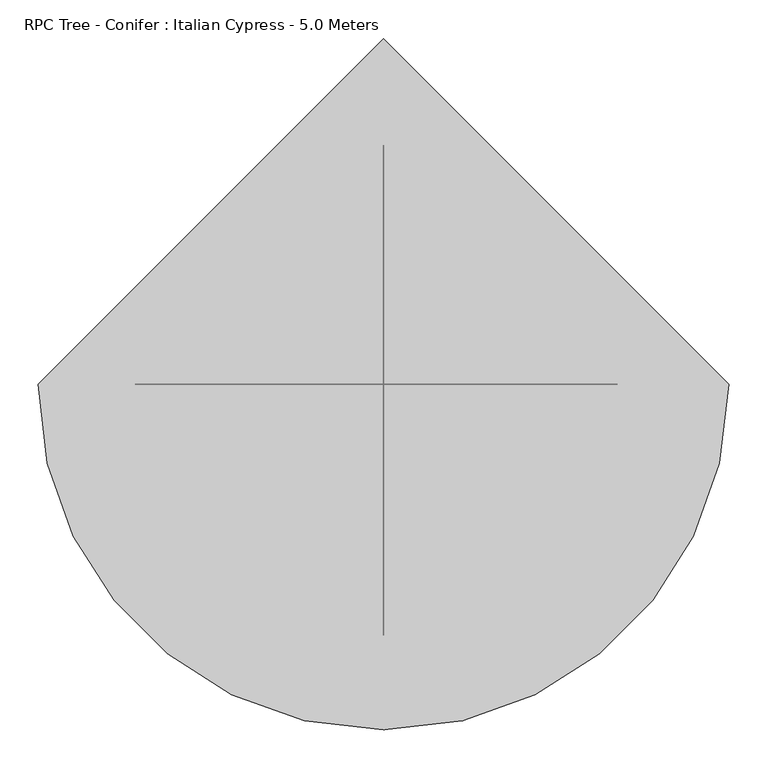
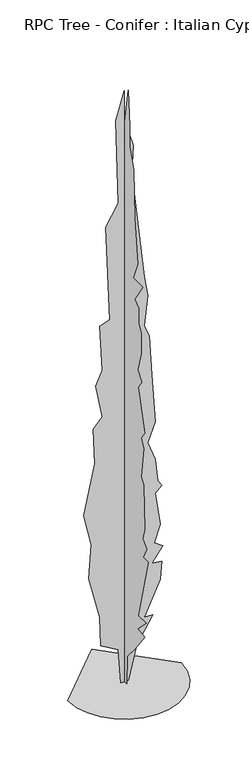
"""IFC4 building model written with IfcOpenShell, lengths in millimetres: geographic element geometry, RPC Tree - Conifer : Italian Cypress - 5.0 Meters."""

from ifc_helpers import new_model, si_unit, origin, place, context, project, spatial, triangles, source, transform, mapped, element, save


def rpc_tree_conifer_italian_cypress_5_0_meters_fed229bb(model_context):
    return source(origin(), model_context, "Body", "Tessellation", [
        triangles([(-28.9243291, 1.3e-06, 0.1175505), (-48.5995771, -1.5e-05, 287.7924989), (-186.3258362, -1.37e-05, 366.4949987), (-196.1633353, -2.79e-05, 612.4350014), (-284.7008453, -4.52e-05, 966.5875122), (-265.0258471, -6.24e-05, 1242.0400303), (-324.0508235, -7.57e-05, 1507.6550674), (-235.513586, -0.0001036, 1910.9949829), (-245.3513394, -0.0001208, 2206.125079), (-176.4880827, -0.0001285, 2284.8250717), (-225.6760869, -0.0001427, 2560.275119), (-176.4880827, -0.0001519, 2678.3248901), (-196.1633353, -0.0001733, 3052.1500374), (-117.4625795, -0.0001785, 3081.6749794), (-146.9753311, -0.0002242, 3868.6749069), (-48.5993273, -0.0002384, 4035.9251633), (-68.2745799, -0.0002792, 4734.3749725), (0.5886036, -0.0002957, 4960.6501144), (0.5885936, -0.0002816, 4724.5499908), (69.4516746, -0.00027, 4478.6001778), (59.614171, -0.0002561, 4252.3500343), (157.9899204, -0.0002064, 3347.2750465), (187.5026721, -0.0001977, 3180.0500793), (157.9899204, -0.0001818, 2934.0999756), (197.3401711, -0.0001776, 2835.7251663), (217.0154237, -0.0001586, 2501.2499428), (246.5281571, -0.0001358, 2097.9100273), (187.5026721, -0.0001239, 1940.5100418), (246.5281571, -0.000117, 1783.1075855), (266.2041727, -0.0001068, 1596.1925411), (295.71667, -0.0001051, 1547.0049911), (246.5281571, -0.0001, 1497.8174412), (285.8791709, -8.53e-05, 1222.3650684), (236.690658, -7.5e-05, 1084.6375013), (305.5541691, -7.51e-05, 1035.450024), (217.0154237, -6.42e-05, 917.4000349), (295.71667, -6.7e-05, 907.5624813), (285.8791709, -5.78e-05, 759.997506), (157.9899204, -3.58e-05, 484.5449879), (226.8529228, -3.88e-05, 484.5449879), (98.9641719, -2.09e-05, 277.9549998), (30.1011696, -1.3e-06, 0.058986), (0.1966738, 26.4907499, 3.55e-05), (0.1966807, 16.6530749, 238.6054939), (0.196685, 95.3537546, 258.2800016), (0.196697, 203.5672438, 494.3825051), (0.1967129, 311.7799882, 819.0225368), (0.1967124, 233.0799954, 887.8875195), (0.1967188, 242.9174945, 1094.4749823), (0.1967282, 272.43001, 1419.1174484), (0.1967333, 262.5925109, 1547.0049911), (0.1967324, 213.4047429, 1645.3799458), (0.1967414, 272.43001, 1861.8075783), (0.1967478, 193.7295085, 2156.9350582), (0.196749, 174.0545104, 2274.9874454), (0.1967577, 223.2422602, 2422.54995), (0.1967593, 164.2167569, 2658.6499283), (0.1967653, 174.054256, 2786.5499702), (0.1967665, 134.7040053, 2924.2749939), (0.1967759, 154.3792578, 3189.875061), (0.1967755, 85.5160011, 3317.775103), (0.1967853, 124.8664971, 3504.675032), (0.19679, 75.678502, 3799.8250397), (0.1967981, 36.3279992, 4094.9500488), (0.1968071, 65.8407486, 4340.8751541), (0.1968079, 26.4905001, 4468.7749054), (0.1968139, -3.0223, 4704.875029), (0.1968216, -52.2102488, 5000.0000381), (0.1968108, -71.8855014, 4704.875029), (0.1968066, -71.8855014, 4537.6250633), (0.1968002, -130.9110046, 4380.2250778), (0.1967852, -140.7485037, 3976.899987), (0.1967737, -180.0987453, 3612.9001122), (0.1967729, -121.0732512, 3465.3251083), (0.1967673, -248.962002, 3465.3251083), (0.1967647, -140.7485037, 3298.1001411), (0.1967635, -199.7739979, 3258.7499268), (0.1967579, -199.7739979, 3130.8498848), (0.1967536, -229.2867495, 3062.0000175), (0.1967493, -229.2867495, 2894.7500519), (0.1967472, -180.0987453, 2727.5250847), (0.1967416, -239.1242486, 2658.6499283), (0.1967438, -189.9364988, 2589.800061), (0.1967284, -278.475008, 2255.3124836), (0.1967275, -229.2867495, 2186.4499718), (0.1967259, -268.6375089, 2117.5849892), (0.1967195, -229.2867495, 1861.8075783), (0.1967156, -268.6375089, 1812.6200283), (0.1967054, -278.475008, 1448.6300365), (0.1967024, -248.9617477, 1350.2524658), (0.1966976, -307.9874871, 1301.0650612), (0.1966986, -258.8000098, 1202.6900339), (0.1966956, -327.6624853, 1202.6900339), (0.1966845, -189.9362444, 671.4600323), (0.1966797, -298.1500062, 671.4600323), (0.1966828, -180.0987453, 553.4074997), (0.1966781, -278.475008, 543.5700188), (0.196679, -150.5860028, 366.4949987), (0.1966781, -42.3724999, 238.6054939), (0.1966712, -32.534751, 3.2e-05), (-450.413314, 0.0, 5.36e-05), (-438.5008143, -103.2502475, 4.7e-05), (-404.5758139, -198.0692509, 3.98e-05), (-351.3483215, -281.7399977, 3.25e-05), (-281.5433345, -351.54751, 2.53e-05), (-197.8723334, -404.7699881, 1.85e-05), (-103.0535753, -438.6974957, 1.23e-05), (0.1966927, -450.6125024, 7.1e-06), (103.4469197, -438.6974957, 3.3e-06), (198.2659141, -404.7724952, 1.1e-06), (281.9366608, -351.5450028, 7e-07), (351.7441913, -281.7399977, 1.8e-06), (404.9666694, -198.0689966, 4.4e-06), (438.894177, -103.2502475, 8.6e-06), (450.8066766, 3.94e-05, 1.42e-05), (0.1966127, 450.6125024, 6.08e-05)], [[17, 18, 19], [39, 40, 41], [16, 17, 19], [16, 19, 20], [16, 20, 21], [16, 21, 22], [15, 16, 22], [14, 15, 22], [14, 22, 23], [14, 23, 24], [34, 35, 36], [36, 37, 38], [42, 1, 2], [41, 42, 2], [39, 41, 2], [30, 31, 32], [39, 2, 3], [39, 3, 4], [38, 39, 4], [36, 38, 4], [36, 4, 5], [34, 36, 5], [34, 5, 6], [33, 34, 6], [32, 33, 6], [32, 6, 7], [32, 7, 8], [30, 32, 8], [29, 30, 8], [28, 29, 8], [28, 8, 9], [27, 28, 9], [27, 9, 10], [26, 27, 10], [26, 10, 11], [26, 11, 12], [25, 26, 12], [25, 12, 13], [24, 25, 13], [14, 24, 13], [67, 68, 69], [94, 95, 96], [74, 75, 76], [96, 97, 98], [92, 93, 94], [100, 43, 44], [99, 100, 44], [67, 69, 70], [66, 67, 70], [66, 70, 71], [65, 66, 71], [65, 71, 72], [64, 65, 72], [63, 64, 72], [63, 72, 73], [62, 63, 73], [62, 73, 74], [61, 62, 74], [61, 74, 76], [90, 91, 92], [81, 82, 83], [46, 47, 48], [60, 61, 76], [59, 60, 76], [59, 76, 77], [59, 77, 78], [59, 78, 79], [59, 79, 80], [59, 80, 81], [58, 59, 81], [57, 58, 81], [57, 81, 83], [56, 57, 83], [56, 83, 84], [55, 56, 84], [55, 84, 85], [54, 55, 85], [53, 54, 85], [53, 85, 86], [53, 86, 87], [52, 53, 87], [52, 87, 88], [52, 88, 89], [51, 52, 89], [51, 89, 90], [50, 51, 90], [49, 50, 90], [49, 90, 92], [49, 92, 94], [48, 49, 94], [46, 48, 94], [46, 94, 96], [46, 96, 98], [45, 46, 98], [45, 98, 99], [44, 45, 99], [115, 116, 101], [114, 115, 101], [114, 101, 102], [113, 114, 102], [113, 102, 103], [113, 103, 104], [112, 113, 104], [111, 112, 104], [111, 104, 105], [111, 105, 106], [111, 106, 107], [111, 107, 108], [111, 108, 109], [111, 109, 110]], closed=False),
    ])


if __name__ == "__main__":
    model = new_model("IFC4")
    model_context = context("Model", 3, world=origin())
    ifc_project = project(units=[si_unit("LENGTHUNIT", "METRE", prefix="MILLI")], contexts=[model_context])
    site = spatial("IfcSite", under=ifc_project)
    building = spatial("IfcBuilding", under=site)
    placement = place(None, origin())
    rpc_tree_conifer_italian_cypress_5_0_meters_shape = rpc_tree_conifer_italian_cypress_5_0_meters_fed229bb(model_context)
    element("IfcGeographicElement", 1, ObjectType="RPC Tree - Conifer : Italian Cypress - 5.0 Meters", at=placement, inside=building, context=model_context, shape_type="MappedRepresentation", body=[
        mapped(rpc_tree_conifer_italian_cypress_5_0_meters_shape, transform((0.0, 0.0, 0.0), x_axis=(1.0, 0.0, 0.0), y_axis=(0.0, 1.0, 0.0), z_axis=(0.0, 0.0, 1.0))),
    ])
    save(model, "model.ifc")

# Revit data of these elements
# Type "RPC Tree - Conifer : Italian Cypress - 5.0 Meters"
#   built-in parameter 1005198 = "{2, 15},{39, RPC-16-FWM7-6P00-C8X0-C000-ST1L-LVER-AU},{1, 0},{1, 0},{2, 13},{1, 8},{5, Color},{1, 0},{1, 0},{3, 0.8},{3, 0.8},{3, 0.8},{1, 8},{7, BBoxMin},{1, 0},{1, 0},{1, 0},{1, 0},{1, 0},{1, 8},{7, BBoxMax},{1, 0},{1, 0},{1, 0},{1, 0},{1, 0},{2, 11},{9, RPCTypeId},{1, 0},{1, 0},{39, RPC-16-FWM7-6P00-C8X0-C000-ST1L-LVER-AU},{1, 6},{14, RPCPlantHeight},{1, 0},{1, 0},{7, 16.4042},{2, 11},{7, keyword},{1, 0},{1, 0},{34, :RPCs:Trees [General]:Geometry:RPC},{2, 11},{8, category},{1, 0},{1, 0},{15, Trees [General]},{2, 11},{12, LocalizedUID},{1, 0},{1, 0},{15, Italian Cypress},{2, 14},{6, Height},{1, 0},{1, 0},{7, 16.4042},{1, 2},{16, Cast Reflections},{1, 0},{1, 0},{1, 0},{1, 2},{12, Cast Shadows},{1, 0},{1, 0},{1, 1},{1, 2},{9, Lock View},{1, 0},{1, 0},{1, 0},{1, 4},{5, ViewC},{1, 0},{1, 0},{1, 0},{21, assetlibrary_base.fbx},{1, 5},"
#   built-in parameter 1005195 = "RPC-16-FWM7-6P00-C8X0-C000-ST1L-LVER-AU"
#   Type Comments = "Italian Cypress"
#   Height = 5000 mm
#   Description = (empty or 0)
